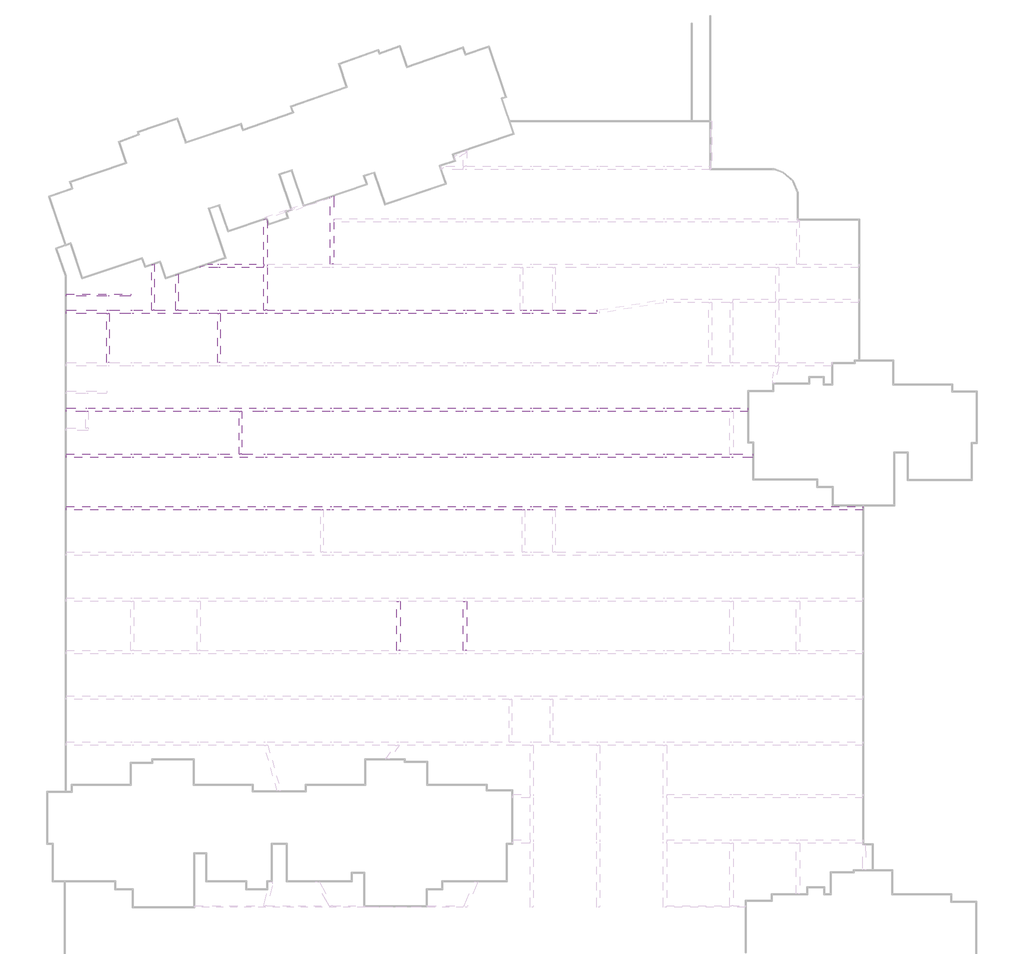
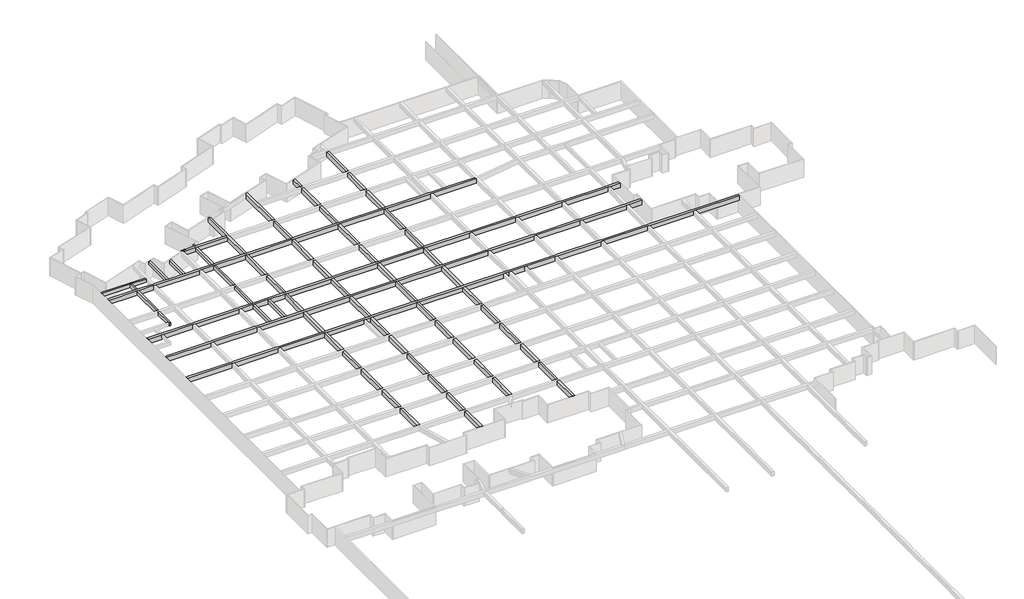
# One storey, part 13 of 14: 15 beams.
"""IFC4 building model written with IfcOpenShell, lengths in millimetres."""

from ifc_helpers import new_model, si_unit, frame, origin, place, context, project, spatial, polyline, outline, extrude, faceted_brep, element, save

model = new_model("IFC4")

# Units and contexts
model_context = context("Model", 3, world=origin())
ifc_project = project(units=[si_unit("LENGTHUNIT", "METRE", prefix="MILLI")], contexts=[model_context])

# Site, building, storey
site = spatial("IfcSite", under=ifc_project)
building = spatial("IfcBuilding", under=site)
storey = spatial("IfcBuildingStorey", under=building, Name="户型图", Elevation=0.0)

# Beams
placement = place(None, origin())
element("IfcBeam", 1, ObjectType="混凝土 - 矩形梁 : KL_beam", at=placement, inside=storey, context=model_context, shape_type="Brep", body=[
    faceted_brep([(-594019.2557706, -38859.4327531, 3300.0), (-594019.2557706, -39259.4327531, 3300.0), (-589117.6529954, -39259.4327531, 3300.0), (-588817.6529954, -39259.4327531, 3300.0), (-586267.6529954, -39259.4327531, 3300.0), (-585867.6529954, -39259.4327531, 3300.0), (-578267.6529954, -39259.4327531, 3300.0), (-577867.6529954, -39259.4327531, 3300.0), (-575817.6529954, -39259.4327531, 3300.0), (-575517.6529954, -39259.4327531, 3300.0), (-570267.6529954, -39259.4327531, 3300.0), (-569867.6529954, -39259.4327531, 3300.0), (-562267.6529954, -39259.4327531, 3300.0), (-561867.6529954, -39259.4327531, 3300.0), (-554267.6529954, -39259.4327531, 3300.0), (-553867.6529954, -39259.4327531, 3300.0), (-546267.6529954, -39259.4327531, 3300.0), (-545867.6529954, -39259.4327531, 3300.0), (-538267.6529954, -39259.4327531, 3300.0), (-537867.6529954, -39259.4327531, 3300.0), (-530267.6529954, -39259.4327531, 3300.0), (-530267.6529954, -38859.4327531, 3300.0), (-535217.6529954, -38859.4327531, 3300.0), (-535517.6529954, -38859.4327531, 3300.0), (-537867.6529954, -38859.4327531, 3300.0), (-538267.6529954, -38859.4327531, 3300.0), (-539117.6529954, -38859.4327531, 3300.0), (-539417.6529954, -38859.4327531, 3300.0), (-545867.6529954, -38859.4327531, 3300.0), (-546267.6529954, -38859.4327531, 3300.0), (-553867.6529954, -38859.4327531, 3300.0), (-554267.6529954, -38859.4327531, 3300.0), (-561867.6529954, -38859.4327531, 3300.0), (-562267.6529954, -38859.4327531, 3300.0), (-569867.6529954, -38859.4327531, 3300.0), (-570267.6529954, -38859.4327531, 3300.0), (-575517.6529954, -38859.4327531, 3300.0), (-575817.6529954, -38859.4327531, 3300.0), (-577867.6529954, -38859.4327531, 3300.0), (-578267.6529954, -38859.4327531, 3300.0), (-580530.3460998, -38859.4327531, 3300.0), (-580830.3460998, -38859.4327531, 3300.0), (-583417.6956186, -38859.4327531, 3300.0), (-583717.6956186, -38859.4327531, 3300.0), (-585867.6529954, -38859.4327531, 3300.0), (-586267.6529954, -38859.4327531, 3300.0), (-588817.6529954, -38859.4327531, 3300.0), (-589117.6529954, -38859.4327531, 3300.0), (-594019.2557706, -39259.4327531, 2500.0), (-586267.6529954, -39259.4327531, 2500.0), (-585867.6529954, -39259.4327531, 2500.0), (-578267.6529954, -39259.4327531, 2500.0), (-577867.6529954, -39259.4327531, 2500.0), (-570267.6529954, -39259.4327531, 2500.0), (-569867.6529954, -39259.4327531, 2500.0), (-562267.6529954, -39259.4327531, 2500.0), (-561867.6529954, -39259.4327531, 2500.0), (-554267.6529954, -39259.4327531, 2500.0), (-553867.6529954, -39259.4327531, 2500.0), (-546267.6529954, -39259.4327531, 2500.0), (-545867.6529954, -39259.4327531, 2500.0), (-538267.6529954, -39259.4327531, 2500.0), (-537867.6529954, -39259.4327531, 2500.0), (-530267.6529954, -39259.4327531, 2500.0), (-594019.2557706, -38859.4327531, 2500.0), (-586267.6529954, -38859.4327531, 2500.0), (-585867.6529954, -38859.4327531, 2500.0), (-578267.6529954, -38859.4327531, 2500.0), (-577867.6529954, -38859.4327531, 2500.0), (-570267.6529954, -38859.4327531, 2500.0), (-569867.6529954, -38859.4327531, 2500.0), (-562267.6529954, -38859.4327531, 2500.0), (-561867.6529954, -38859.4327531, 2500.0), (-554267.6529954, -38859.4327531, 2500.0), (-553867.6529954, -38859.4327531, 2500.0), (-546267.6529954, -38859.4327531, 2500.0), (-545867.6529954, -38859.4327531, 2500.0), (-538267.6529954, -38859.4327531, 2500.0), (-537867.6529954, -38859.4327531, 2500.0), (-530267.6529954, -38859.4327531, 2500.0)], [[[0, 1, 2, 3, 4, 5, 6, 7, 8, 9, 10, 11, 12, 13, 14, 15, 16, 17, 18, 19, 20, 21, 22, 23, 24, 25, 26, 27, 28, 29, 30, 31, 32, 33, 34, 35, 36, 37, 38, 39, 40, 41, 42, 43, 44, 45, 46, 47]], [[1, 48, 49, 50, 51, 52, 53, 54, 55, 56, 57, 58, 59, 60, 61, 62, 63, 20, 19, 18, 17, 16, 15, 14, 13, 12, 11, 10, 9, 8, 7, 6, 5, 4, 3, 2]], [[48, 64, 65, 66, 67, 68, 69, 70, 71, 72, 73, 74, 75, 76, 77, 78, 79, 63, 62, 61, 60, 59, 58, 57, 56, 55, 54, 53, 52, 51, 50, 49]], [[64, 0, 47, 46, 45, 44, 43, 42, 41, 40, 39, 38, 37, 36, 35, 34, 33, 32, 31, 30, 29, 28, 27, 26, 25, 24, 23, 22, 21, 79, 78, 77, 76, 75, 74, 73, 72, 71, 70, 69, 68, 67, 66, 65]], [[1, 0, 64, 48]], [[21, 20, 63, 79]]]),
])
element("IfcBeam", 2, ObjectType="混凝土 - 矩形梁 : KL_beam", at=placement, inside=storey, context=model_context, shape_type="Brep", body=[
    faceted_brep([(-594019.2557706, -56159.4327531, 3300.0), (-594019.2557706, -56559.4327531, 3300.0), (-586267.6529954, -56559.4327531, 3300.0), (-585867.6529954, -56559.4327531, 3300.0), (-578267.6529954, -56559.4327531, 3300.0), (-577867.6529954, -56559.4327531, 3300.0), (-570267.6529954, -56559.4327531, 3300.0), (-569867.6529954, -56559.4327531, 3300.0), (-562267.6529954, -56559.4327531, 3300.0), (-561867.6529954, -56559.4327531, 3300.0), (-554267.6529954, -56559.4327531, 3300.0), (-553867.6529954, -56559.4327531, 3300.0), (-546267.6529954, -56559.4327531, 3300.0), (-545867.6529954, -56559.4327531, 3300.0), (-538267.6529954, -56559.4327531, 3300.0), (-537867.6529954, -56559.4327531, 3300.0), (-530267.6529954, -56559.4327531, 3300.0), (-529867.6529954, -56559.4327531, 3300.0), (-522267.6529954, -56559.4327531, 3300.0), (-521867.6529954, -56559.4327531, 3300.0), (-514267.6529954, -56559.4327531, 3300.0), (-513867.6529954, -56559.4327531, 3300.0), (-511515.1621146, -56559.4327531, 3300.0), (-511515.1621146, -56159.4327531, 3300.0), (-513867.6529954, -56159.4327531, 3300.0), (-514267.6529954, -56159.4327531, 3300.0), (-521867.6529954, -56159.4327531, 3300.0), (-522267.6529954, -56159.4327531, 3300.0), (-529867.6529954, -56159.4327531, 3300.0), (-530267.6529954, -56159.4327531, 3300.0), (-537867.6529954, -56159.4327531, 3300.0), (-538267.6529954, -56159.4327531, 3300.0), (-545867.6529954, -56159.4327531, 3300.0), (-546267.6529954, -56159.4327531, 3300.0), (-553867.6529954, -56159.4327531, 3300.0), (-554267.6529954, -56159.4327531, 3300.0), (-561867.6529954, -56159.4327531, 3300.0), (-562267.6529954, -56159.4327531, 3300.0), (-569867.6529954, -56159.4327531, 3300.0), (-570267.6529954, -56159.4327531, 3300.0), (-572917.6529954, -56159.4327531, 3300.0), (-573217.6529954, -56159.4327531, 3300.0), (-575517.6529954, -56159.4327531, 3300.0), (-575817.6529954, -56159.4327531, 3300.0), (-577867.6529954, -56159.4327531, 3300.0), (-578267.6529954, -56159.4327531, 3300.0), (-585867.6529954, -56159.4327531, 3300.0), (-586267.6529954, -56159.4327531, 3300.0), (-594019.2557706, -56559.4327531, 2500.0), (-586267.6529954, -56559.4327531, 2500.0), (-585867.6529954, -56559.4327531, 2500.0), (-578267.6529954, -56559.4327531, 2500.0), (-577867.6529954, -56559.4327531, 2500.0), (-570267.6529954, -56559.4327531, 2500.0), (-569867.6529954, -56559.4327531, 2500.0), (-562267.6529954, -56559.4327531, 2500.0), (-561867.6529954, -56559.4327531, 2500.0), (-554267.6529954, -56559.4327531, 2500.0), (-553867.6529954, -56559.4327531, 2500.0), (-546267.6529954, -56559.4327531, 2500.0), (-545867.6529954, -56559.4327531, 2500.0), (-538267.6529954, -56559.4327531, 2500.0), (-537867.6529954, -56559.4327531, 2500.0), (-530267.6529954, -56559.4327531, 2500.0), (-529867.6529954, -56559.4327531, 2500.0), (-522267.6529954, -56559.4327531, 2500.0), (-521867.6529954, -56559.4327531, 2500.0), (-514267.6529954, -56559.4327531, 2500.0), (-513867.6529954, -56559.4327531, 2500.0), (-511515.1621146, -56559.4327531, 2500.0), (-594019.2557706, -56159.4327531, 2500.0), (-586267.6529954, -56159.4327531, 2500.0), (-585867.6529954, -56159.4327531, 2500.0), (-578267.6529954, -56159.4327531, 2500.0), (-577867.6529954, -56159.4327531, 2500.0), (-570267.6529954, -56159.4327531, 2500.0), (-569867.6529954, -56159.4327531, 2500.0), (-562267.6529954, -56159.4327531, 2500.0), (-561867.6529954, -56159.4327531, 2500.0), (-554267.6529954, -56159.4327531, 2500.0), (-553867.6529954, -56159.4327531, 2500.0), (-546267.6529954, -56159.4327531, 2500.0), (-545867.6529954, -56159.4327531, 2500.0), (-538267.6529954, -56159.4327531, 2500.0), (-537867.6529954, -56159.4327531, 2500.0), (-530267.6529954, -56159.4327531, 2500.0), (-529867.6529954, -56159.4327531, 2500.0), (-522267.6529954, -56159.4327531, 2500.0), (-521867.6529954, -56159.4327531, 2500.0), (-514267.6529954, -56159.4327531, 2500.0), (-513867.6529954, -56159.4327531, 2500.0), (-511515.1621146, -56159.4327531, 2500.0)], [[[0, 1, 2, 3, 4, 5, 6, 7, 8, 9, 10, 11, 12, 13, 14, 15, 16, 17, 18, 19, 20, 21, 22, 23, 24, 25, 26, 27, 28, 29, 30, 31, 32, 33, 34, 35, 36, 37, 38, 39, 40, 41, 42, 43, 44, 45, 46, 47]], [[1, 48, 49, 50, 51, 52, 53, 54, 55, 56, 57, 58, 59, 60, 61, 62, 63, 64, 65, 66, 67, 68, 69, 22, 21, 20, 19, 18, 17, 16, 15, 14, 13, 12, 11, 10, 9, 8, 7, 6, 5, 4, 3, 2]], [[48, 70, 71, 72, 73, 74, 75, 76, 77, 78, 79, 80, 81, 82, 83, 84, 85, 86, 87, 88, 89, 90, 91, 69, 68, 67, 66, 65, 64, 63, 62, 61, 60, 59, 58, 57, 56, 55, 54, 53, 52, 51, 50, 49]], [[70, 0, 47, 46, 45, 44, 43, 42, 41, 40, 39, 38, 37, 36, 35, 34, 33, 32, 31, 30, 29, 28, 27, 26, 25, 24, 23, 91, 90, 89, 88, 87, 86, 85, 84, 83, 82, 81, 80, 79, 78, 77, 76, 75, 74, 73, 72, 71]], [[1, 0, 70, 48]], [[23, 22, 69, 91]]]),
])
element("IfcBeam", 3, ObjectType="混凝土 - 矩形梁 : KL_beam", at=placement, inside=storey, context=model_context, shape_type="Brep", body=[
    faceted_brep([(-594019.2557706, -50659.4327531, 3300.0), (-594019.2557706, -51059.4327531, 3300.0), (-591673.454383, -51059.4327531, 3300.0), (-591373.454383, -51059.4327531, 3300.0), (-586267.6529954, -51059.4327531, 3300.0), (-585867.6529954, -51059.4327531, 3300.0), (-578267.6529954, -51059.4327531, 3300.0), (-577867.6529954, -51059.4327531, 3300.0), (-575817.6529954, -51059.4327531, 3300.0), (-575517.6529954, -51059.4327531, 3300.0), (-573217.6529954, -51059.4327531, 3300.0), (-572917.6529954, -51059.4327531, 3300.0), (-570267.6529954, -51059.4327531, 3300.0), (-569867.6529954, -51059.4327531, 3300.0), (-562267.6529954, -51059.4327531, 3300.0), (-561867.6529954, -51059.4327531, 3300.0), (-554267.6529954, -51059.4327531, 3300.0), (-553867.6529954, -51059.4327531, 3300.0), (-546267.6529954, -51059.4327531, 3300.0), (-545867.6529954, -51059.4327531, 3300.0), (-538267.6529954, -51059.4327531, 3300.0), (-537867.6529954, -51059.4327531, 3300.0), (-530267.6529954, -51059.4327531, 3300.0), (-529867.6529954, -51059.4327531, 3300.0), (-522267.6529954, -51059.4327531, 3300.0), (-521867.6529954, -51059.4327531, 3300.0), (-514267.6529954, -51059.4327531, 3300.0), (-513867.6529954, -51059.4327531, 3300.0), (-512115.1621146, -51059.4327531, 3300.0), (-512115.1621146, -50659.4327531, 3300.0), (-513867.6529954, -50659.4327531, 3300.0), (-514267.6529954, -50659.4327531, 3300.0), (-521867.6529954, -50659.4327531, 3300.0), (-522267.6529954, -50659.4327531, 3300.0), (-529867.6529954, -50659.4327531, 3300.0), (-530267.6529954, -50659.4327531, 3300.0), (-537867.6529954, -50659.4327531, 3300.0), (-538267.6529954, -50659.4327531, 3300.0), (-545867.6529954, -50659.4327531, 3300.0), (-546267.6529954, -50659.4327531, 3300.0), (-553867.6529954, -50659.4327531, 3300.0), (-554267.6529954, -50659.4327531, 3300.0), (-561867.6529954, -50659.4327531, 3300.0), (-562267.6529954, -50659.4327531, 3300.0), (-569867.6529954, -50659.4327531, 3300.0), (-570267.6529954, -50659.4327531, 3300.0), (-575517.6529954, -50659.4327531, 3300.0), (-575817.6529954, -50659.4327531, 3300.0), (-577867.6529954, -50659.4327531, 3300.0), (-578267.6529954, -50659.4327531, 3300.0), (-585867.6529954, -50659.4327531, 3300.0), (-586267.6529954, -50659.4327531, 3300.0), (-591373.454383, -50659.4327531, 3300.0), (-591673.454383, -50659.4327531, 3300.0), (-594019.2557706, -51059.4327531, 2500.0), (-586267.6529954, -51059.4327531, 2500.0), (-585867.6529954, -51059.4327531, 2500.0), (-578267.6529954, -51059.4327531, 2500.0), (-577867.6529954, -51059.4327531, 2500.0), (-570267.6529954, -51059.4327531, 2500.0), (-569867.6529954, -51059.4327531, 2500.0), (-562267.6529954, -51059.4327531, 2500.0), (-561867.6529954, -51059.4327531, 2500.0), (-554267.6529954, -51059.4327531, 2500.0), (-553867.6529954, -51059.4327531, 2500.0), (-546267.6529954, -51059.4327531, 2500.0), (-545867.6529954, -51059.4327531, 2500.0), (-538267.6529954, -51059.4327531, 2500.0), (-537867.6529954, -51059.4327531, 2500.0), (-530267.6529954, -51059.4327531, 2500.0), (-529867.6529954, -51059.4327531, 2500.0), (-522267.6529954, -51059.4327531, 2500.0), (-521867.6529954, -51059.4327531, 2500.0), (-514267.6529954, -51059.4327531, 2500.0), (-513867.6529954, -51059.4327531, 2500.0), (-512115.1621146, -51059.4327531, 2500.0), (-594019.2557706, -50659.4327531, 2500.0), (-586267.6529954, -50659.4327531, 2500.0), (-585867.6529954, -50659.4327531, 2500.0), (-578267.6529954, -50659.4327531, 2500.0), (-577867.6529954, -50659.4327531, 2500.0), (-570267.6529954, -50659.4327531, 2500.0), (-569867.6529954, -50659.4327531, 2500.0), (-562267.6529954, -50659.4327531, 2500.0), (-561867.6529954, -50659.4327531, 2500.0), (-554267.6529954, -50659.4327531, 2500.0), (-553867.6529954, -50659.4327531, 2500.0), (-546267.6529954, -50659.4327531, 2500.0), (-545867.6529954, -50659.4327531, 2500.0), (-538267.6529954, -50659.4327531, 2500.0), (-537867.6529954, -50659.4327531, 2500.0), (-530267.6529954, -50659.4327531, 2500.0), (-529867.6529954, -50659.4327531, 2500.0), (-522267.6529954, -50659.4327531, 2500.0), (-521867.6529954, -50659.4327531, 2500.0), (-514267.6529954, -50659.4327531, 2500.0), (-513867.6529954, -50659.4327531, 2500.0), (-512115.1621146, -50659.4327531, 2500.0)], [[[0, 1, 2, 3, 4, 5, 6, 7, 8, 9, 10, 11, 12, 13, 14, 15, 16, 17, 18, 19, 20, 21, 22, 23, 24, 25, 26, 27, 28, 29, 30, 31, 32, 33, 34, 35, 36, 37, 38, 39, 40, 41, 42, 43, 44, 45, 46, 47, 48, 49, 50, 51, 52, 53]], [[1, 54, 55, 56, 57, 58, 59, 60, 61, 62, 63, 64, 65, 66, 67, 68, 69, 70, 71, 72, 73, 74, 75, 28, 27, 26, 25, 24, 23, 22, 21, 20, 19, 18, 17, 16, 15, 14, 13, 12, 11, 10, 9, 8, 7, 6, 5, 4, 3, 2]], [[54, 76, 77, 78, 79, 80, 81, 82, 83, 84, 85, 86, 87, 88, 89, 90, 91, 92, 93, 94, 95, 96, 97, 75, 74, 73, 72, 71, 70, 69, 68, 67, 66, 65, 64, 63, 62, 61, 60, 59, 58, 57, 56, 55]], [[76, 0, 53, 52, 51, 50, 49, 48, 47, 46, 45, 44, 43, 42, 41, 40, 39, 38, 37, 36, 35, 34, 33, 32, 31, 30, 29, 97, 96, 95, 94, 93, 92, 91, 90, 89, 88, 87, 86, 85, 84, 83, 82, 81, 80, 79, 78, 77]], [[1, 0, 76, 54]], [[29, 28, 75, 97]]]),
])
element("IfcBeam", 4, ObjectType="混凝土 - 矩形梁 : KL_beam", at=placement, inside=storey, context=model_context, shape_type="Brep", body=[
    faceted_brep([(-594019.2557706, -62459.4327531, 3300.0), (-594019.2557706, -62859.4327531, 3300.0), (-586267.6529954, -62859.4327531, 3300.0), (-585867.6529954, -62859.4327531, 3300.0), (-578267.6529954, -62859.4327531, 3300.0), (-577867.6529954, -62859.4327531, 3300.0), (-570267.6529954, -62859.4327531, 3300.0), (-569867.6529954, -62859.4327531, 3300.0), (-563417.6529954, -62859.4327531, 3300.0), (-563117.6529954, -62859.4327531, 3300.0), (-562267.6529954, -62859.4327531, 3300.0), (-561867.6529954, -62859.4327531, 3300.0), (-554267.6529954, -62859.4327531, 3300.0), (-553867.6529954, -62859.4327531, 3300.0), (-546267.6529954, -62859.4327531, 3300.0), (-545867.6529954, -62859.4327531, 3300.0), (-539217.6529954, -62859.4327531, 3300.0), (-538917.6529954, -62859.4327531, 3300.0), (-538267.6529954, -62859.4327531, 3300.0), (-537867.6529954, -62859.4327531, 3300.0), (-535517.6529954, -62859.4327531, 3300.0), (-535217.6529954, -62859.4327531, 3300.0), (-530267.6529954, -62859.4327531, 3300.0), (-529867.6529954, -62859.4327531, 3300.0), (-522267.6529954, -62859.4327531, 3300.0), (-521867.6529954, -62859.4327531, 3300.0), (-514267.6529954, -62859.4327531, 3300.0), (-513867.6529954, -62859.4327531, 3300.0), (-506267.6529954, -62859.4327531, 3300.0), (-505867.6529954, -62859.4327531, 3300.0), (-498277.6529954, -62859.4327531, 3300.0), (-498277.6529954, -62459.4327531, 3300.0), (-505867.6529954, -62459.4327531, 3300.0), (-506267.6529954, -62459.4327531, 3300.0), (-513867.6529954, -62459.4327531, 3300.0), (-514267.6529954, -62459.4327531, 3300.0), (-521867.6529954, -62459.4327531, 3300.0), (-522267.6529954, -62459.4327531, 3300.0), (-529867.6529954, -62459.4327531, 3300.0), (-530267.6529954, -62459.4327531, 3300.0), (-537867.6529954, -62459.4327531, 3300.0), (-538267.6529954, -62459.4327531, 3300.0), (-545867.6529954, -62459.4327531, 3300.0), (-546267.6529954, -62459.4327531, 3300.0), (-553867.6529954, -62459.4327531, 3300.0), (-554267.6529954, -62459.4327531, 3300.0), (-561867.6529954, -62459.4327531, 3300.0), (-562267.6529954, -62459.4327531, 3300.0), (-569867.6529954, -62459.4327531, 3300.0), (-570267.6529954, -62459.4327531, 3300.0), (-577867.6529954, -62459.4327531, 3300.0), (-578267.6529954, -62459.4327531, 3300.0), (-585867.6529954, -62459.4327531, 3300.0), (-586267.6529954, -62459.4327531, 3300.0), (-594019.2557706, -62859.4327531, 2500.0), (-586267.6529954, -62859.4327531, 2500.0), (-585867.6529954, -62859.4327531, 2500.0), (-578267.6529954, -62859.4327531, 2500.0), (-577867.6529954, -62859.4327531, 2500.0), (-570267.6529954, -62859.4327531, 2500.0), (-569867.6529954, -62859.4327531, 2500.0), (-562267.6529954, -62859.4327531, 2500.0), (-561867.6529954, -62859.4327531, 2500.0), (-554267.6529954, -62859.4327531, 2500.0), (-553867.6529954, -62859.4327531, 2500.0), (-546267.6529954, -62859.4327531, 2500.0), (-545867.6529954, -62859.4327531, 2500.0), (-538267.6529954, -62859.4327531, 2500.0), (-537867.6529954, -62859.4327531, 2500.0), (-530267.6529954, -62859.4327531, 2500.0), (-529867.6529954, -62859.4327531, 2500.0), (-522267.6529954, -62859.4327531, 2500.0), (-521867.6529954, -62859.4327531, 2500.0), (-514267.6529954, -62859.4327531, 2500.0), (-513867.6529954, -62859.4327531, 2500.0), (-506267.6529954, -62859.4327531, 2500.0), (-505867.6529954, -62859.4327531, 2500.0), (-498277.6529954, -62859.4327531, 2500.0), (-594019.2557706, -62459.4327531, 2500.0), (-586267.6529954, -62459.4327531, 2500.0), (-585867.6529954, -62459.4327531, 2500.0), (-578267.6529954, -62459.4327531, 2500.0), (-577867.6529954, -62459.4327531, 2500.0), (-570267.6529954, -62459.4327531, 2500.0), (-569867.6529954, -62459.4327531, 2500.0), (-562267.6529954, -62459.4327531, 2500.0), (-561867.6529954, -62459.4327531, 2500.0), (-554267.6529954, -62459.4327531, 2500.0), (-553867.6529954, -62459.4327531, 2500.0), (-546267.6529954, -62459.4327531, 2500.0), (-545867.6529954, -62459.4327531, 2500.0), (-538267.6529954, -62459.4327531, 2500.0), (-537867.6529954, -62459.4327531, 2500.0), (-530267.6529954, -62459.4327531, 2500.0), (-529867.6529954, -62459.4327531, 2500.0), (-522267.6529954, -62459.4327531, 2500.0), (-521867.6529954, -62459.4327531, 2500.0), (-514267.6529954, -62459.4327531, 2500.0), (-513867.6529954, -62459.4327531, 2500.0), (-506267.6529954, -62459.4327531, 2500.0), (-505867.6529954, -62459.4327531, 2500.0), (-498277.6529954, -62459.4327531, 2500.0)], [[[0, 1, 2, 3, 4, 5, 6, 7, 8, 9, 10, 11, 12, 13, 14, 15, 16, 17, 18, 19, 20, 21, 22, 23, 24, 25, 26, 27, 28, 29, 30, 31, 32, 33, 34, 35, 36, 37, 38, 39, 40, 41, 42, 43, 44, 45, 46, 47, 48, 49, 50, 51, 52, 53]], [[1, 54, 55, 56, 57, 58, 59, 60, 61, 62, 63, 64, 65, 66, 67, 68, 69, 70, 71, 72, 73, 74, 75, 76, 77, 30, 29, 28, 27, 26, 25, 24, 23, 22, 21, 20, 19, 18, 17, 16, 15, 14, 13, 12, 11, 10, 9, 8, 7, 6, 5, 4, 3, 2]], [[54, 78, 79, 80, 81, 82, 83, 84, 85, 86, 87, 88, 89, 90, 91, 92, 93, 94, 95, 96, 97, 98, 99, 100, 101, 77, 76, 75, 74, 73, 72, 71, 70, 69, 68, 67, 66, 65, 64, 63, 62, 61, 60, 59, 58, 57, 56, 55]], [[78, 0, 53, 52, 51, 50, 49, 48, 47, 46, 45, 44, 43, 42, 41, 40, 39, 38, 37, 36, 35, 34, 33, 32, 31, 101, 100, 99, 98, 97, 96, 95, 94, 93, 92, 91, 90, 89, 88, 87, 86, 85, 84, 83, 82, 81, 80, 79]], [[1, 0, 78, 54]], [[31, 30, 77, 101]]]),
])
element("IfcBeam", 5, ObjectType="混凝土 - 矩形梁 : KL_beam", at=placement, inside=storey, context=model_context, shape_type="Brep", body=[
    faceted_brep([(-569950.4085273, -27888.1137818, 3300.0), (-570267.6529954, -27994.502473, 3300.0), (-570267.6529954, -33359.4327531, 3300.0), (-570267.6529954, -33759.4327531, 3300.0), (-570267.6529954, -38859.4327531, 3300.0), (-569867.6529954, -38859.4327531, 3300.0), (-569867.6529954, -33759.4327531, 3300.0), (-569867.6529954, -33359.4327531, 3300.0), (-569867.6529954, -28133.2700068, 3300.0), (-569867.6529954, -28133.2700068, 2500.0), (-569867.6529954, -38859.4327531, 2500.0), (-569867.6529954, -33759.4327531, 2500.0), (-569867.6529954, -33359.4327531, 2500.0), (-570267.6529954, -27994.502473, 2500.0), (-569950.4085273, -27888.1137818, 2500.0), (-570267.6529954, -38859.4327531, 2500.0), (-570267.6529954, -33759.4327531, 2500.0), (-570267.6529954, -33359.4327531, 2500.0)], [[[0, 1, 2, 3, 4, 5, 6, 7, 8]], [[9, 8, 7, 6, 5, 10, 11, 12]], [[13, 14, 9, 12, 11, 10, 15, 16, 17]], [[1, 13, 17, 16, 15, 4, 3, 2]], [[13, 1, 0, 14]], [[14, 0, 8, 9]], [[4, 15, 10, 5]]]),
    faceted_brep([(-570267.6529954, -90759.4327531, 3300.0), (-570267.6529954, -90759.4327531, 2500.0), (-569867.6529954, -90759.4327531, 2500.0), (-569867.6529954, -90759.4327531, 3300.0), (-570267.6529954, -85659.4327531, 2500.0), (-570267.6529954, -85659.4327531, 3300.0), (-569867.6529954, -85659.4327531, 3300.0), (-569867.6529954, -85659.4327531, 2500.0)], [[[0, 1, 2, 3]], [[4, 5, 6, 7]], [[1, 0, 5, 4]], [[0, 3, 6, 5]], [[3, 2, 7, 6]], [[2, 1, 4, 7]]]),
    faceted_brep([(-570267.6529954, -39259.4327531, 2500.0), (-570267.6529954, -39259.4327531, 3300.0), (-569867.6529954, -39259.4327531, 3300.0), (-569867.6529954, -39259.4327531, 2500.0), (-570267.6529954, -45159.4327531, 2500.0), (-570267.6529954, -45159.4327531, 3300.0), (-569867.6529954, -45159.4327531, 2500.0), (-569867.6529954, -45159.4327531, 3300.0)], [[[0, 1, 2, 3]], [[1, 0, 4, 5]], [[5, 4, 6, 7]], [[2, 1, 5, 7]], [[3, 2, 7, 6]], [[0, 3, 6, 4]]]),
    faceted_brep([(-570267.6529954, -45559.4327531, 2500.0), (-570267.6529954, -45559.4327531, 3300.0), (-569867.6529954, -45559.4327531, 3300.0), (-569867.6529954, -45559.4327531, 2500.0), (-570267.6529954, -50659.4327531, 2500.0), (-570267.6529954, -50659.4327531, 3300.0), (-569867.6529954, -50659.4327531, 2500.0), (-569867.6529954, -50659.4327531, 3300.0)], [[[0, 1, 2, 3]], [[1, 0, 4, 5]], [[5, 4, 6, 7]], [[2, 1, 5, 7]], [[3, 2, 7, 6]], [[0, 3, 6, 4]]]),
    faceted_brep([(-570267.6529954, -56559.4327531, 2500.0), (-570267.6529954, -56559.4327531, 3300.0), (-569867.6529954, -56559.4327531, 3300.0), (-569867.6529954, -56559.4327531, 2500.0), (-570267.6529954, -62459.4327531, 2500.0), (-570267.6529954, -62459.4327531, 3300.0), (-569867.6529954, -62459.4327531, 2500.0), (-569867.6529954, -62459.4327531, 3300.0)], [[[0, 1, 2, 3]], [[1, 0, 4, 5]], [[5, 4, 6, 7]], [[2, 1, 5, 7]], [[3, 2, 7, 6]], [[0, 3, 6, 4]]]),
    faceted_brep([(-570267.6529954, -56159.4327531, 3300.0), (-570267.6529954, -56159.4327531, 2500.0), (-569867.6529954, -56159.4327531, 2500.0), (-569867.6529954, -56159.4327531, 3300.0), (-570267.6529954, -51059.4327531, 2500.0), (-570267.6529954, -51059.4327531, 3300.0), (-569867.6529954, -51059.4327531, 3300.0), (-569867.6529954, -51059.4327531, 2500.0)], [[[0, 1, 2, 3]], [[4, 5, 6, 7]], [[1, 0, 5, 4]], [[0, 3, 6, 5]], [[3, 2, 7, 6]], [[2, 1, 4, 7]]]),
    faceted_brep([(-570267.6529954, -62859.4327531, 2500.0), (-570267.6529954, -62859.4327531, 3300.0), (-569867.6529954, -62859.4327531, 3300.0), (-569867.6529954, -62859.4327531, 2500.0), (-570267.6529954, -67959.4327531, 2500.0), (-570267.6529954, -67959.4327531, 3300.0), (-569867.6529954, -67959.4327531, 2500.0), (-569867.6529954, -67959.4327531, 3300.0)], [[[0, 1, 2, 3]], [[1, 0, 4, 5]], [[5, 4, 6, 7]], [[2, 1, 5, 7]], [[3, 2, 7, 6]], [[0, 3, 6, 4]]]),
    faceted_brep([(-570267.6529954, -68359.4327531, 2500.0), (-570267.6529954, -68359.4327531, 3300.0), (-569867.6529954, -68359.4327531, 3300.0), (-569867.6529954, -68359.4327531, 2500.0), (-570267.6529954, -73459.4327531, 2500.0), (-570267.6529954, -73459.4327531, 3300.0), (-569867.6529954, -73459.4327531, 2500.0), (-569867.6529954, -73459.4327531, 3300.0)], [[[0, 1, 2, 3]], [[1, 0, 4, 5]], [[5, 4, 6, 7]], [[2, 1, 5, 7]], [[3, 2, 7, 6]], [[0, 3, 6, 4]]]),
    faceted_brep([(-570267.6529954, -73859.4327531, 2500.0), (-570267.6529954, -73859.4327531, 3300.0), (-569867.6529954, -73859.4327531, 3300.0), (-569867.6529954, -73859.4327531, 2500.0), (-570267.6529954, -79759.4327531, 2500.0), (-570267.6529954, -79759.4327531, 3300.0), (-569867.6529954, -79759.4327531, 2500.0), (-569867.6529954, -79759.4327531, 3300.0)], [[[0, 1, 2, 3]], [[1, 0, 4, 5]], [[5, 4, 6, 7]], [[2, 1, 5, 7]], [[3, 2, 7, 6]], [[0, 3, 6, 4]]]),
    faceted_brep([(-570267.6529954, -80159.4327531, 2500.0), (-570267.6529954, -80159.4327531, 3300.0), (-569867.6529954, -80159.4327531, 3300.0), (-569867.6529954, -80159.4327531, 2500.0), (-570267.6529954, -85259.4327531, 2500.0), (-570267.6529954, -85259.4327531, 3300.0), (-569867.6529954, -85259.4327531, 2500.0), (-569867.6529954, -85259.4327531, 3300.0)], [[[0, 1, 2, 3]], [[1, 0, 4, 5]], [[5, 4, 6, 7]], [[2, 1, 5, 7]], [[3, 2, 7, 6]], [[0, 3, 6, 4]]]),
])
element("IfcBeam", 6, ObjectType="混凝土 - 矩形梁 : KL_beam", at=placement, inside=storey, context=model_context, shape_type="Brep", body=[
    faceted_brep([(-561867.6529954, -25159.8064152, 3300.0), (-562267.6529954, -25294.8313886, 3300.0), (-562267.6529954, -25442.5926439, 3300.0), (-562267.6529954, -33359.4327531, 3300.0), (-561867.6529954, -33359.4327531, 3300.0), (-561867.6529954, -28259.4327531, 3300.0), (-561867.6529954, -27859.4327531, 3300.0), (-562267.6529954, -25294.8313886, 2500.0), (-562267.6529954, -25442.5926439, 2500.0), (-562267.6529954, -33359.4327531, 2500.0), (-561867.6529954, -25159.8064152, 2500.0), (-561867.6529954, -27859.4327531, 2500.0), (-561867.6529954, -28259.4327531, 2500.0), (-561867.6529954, -33359.4327531, 2500.0)], [[[0, 1, 2, 3, 4, 5, 6]], [[1, 7, 8, 9, 3, 2]], [[7, 10, 11, 12, 13, 9, 8]], [[10, 0, 6, 5, 4, 13, 12, 11]], [[1, 0, 10, 7]], [[4, 3, 9, 13]]]),
    faceted_brep([(-561867.6529954, -95855.8355501, 3300.0), (-562267.6529954, -95855.8355501, 3300.0), (-562267.6529954, -95855.8355501, 2500.0), (-561867.6529954, -95855.8355501, 2500.0), (-561867.6529954, -91159.4327531, 3300.0), (-562267.6529954, -91159.4327531, 3300.0), (-562267.6529954, -91159.4327531, 2500.0), (-561867.6529954, -91159.4327531, 2500.0)], [[[0, 1, 2, 3]], [[1, 0, 4, 5]], [[2, 1, 5, 6]], [[3, 2, 6, 7]], [[0, 3, 7, 4]], [[5, 4, 7, 6]]]),
    faceted_brep([(-562267.6529954, -33759.4327531, 3300.0), (-561867.6529954, -33759.4327531, 3300.0), (-561867.6529954, -33759.4327531, 2500.0), (-562267.6529954, -33759.4327531, 2500.0), (-561867.6529954, -38859.4327531, 3300.0), (-562267.6529954, -38859.4327531, 3300.0), (-562267.6529954, -38859.4327531, 2500.0), (-561867.6529954, -38859.4327531, 2500.0)], [[[0, 1, 2, 3]], [[4, 5, 6, 7]], [[1, 0, 5, 4]], [[0, 3, 6, 5]], [[3, 2, 7, 6]], [[2, 1, 4, 7]]]),
    faceted_brep([(-561867.6529954, -39259.4327531, 3300.0), (-562267.6529954, -39259.4327531, 3300.0), (-562267.6529954, -45159.4327531, 3300.0), (-561867.6529954, -45159.4327531, 3300.0), (-562267.6529954, -39259.4327531, 2500.0), (-562267.6529954, -45159.4327531, 2500.0), (-561867.6529954, -39259.4327531, 2500.0), (-561867.6529954, -45159.4327531, 2500.0)], [[[0, 1, 2, 3]], [[1, 4, 5, 2]], [[4, 6, 7, 5]], [[6, 0, 3, 7]], [[1, 0, 6, 4]], [[3, 2, 5, 7]]]),
    faceted_brep([(-562267.6529954, -45559.4327531, 3300.0), (-561867.6529954, -45559.4327531, 3300.0), (-561867.6529954, -45559.4327531, 2500.0), (-562267.6529954, -45559.4327531, 2500.0), (-561867.6529954, -50659.4327531, 3300.0), (-562267.6529954, -50659.4327531, 3300.0), (-562267.6529954, -50659.4327531, 2500.0), (-561867.6529954, -50659.4327531, 2500.0)], [[[0, 1, 2, 3]], [[4, 5, 6, 7]], [[1, 0, 5, 4]], [[0, 3, 6, 5]], [[3, 2, 7, 6]], [[2, 1, 4, 7]]]),
    faceted_brep([(-561867.6529954, -56559.4327531, 3300.0), (-562267.6529954, -56559.4327531, 3300.0), (-562267.6529954, -62459.4327531, 3300.0), (-561867.6529954, -62459.4327531, 3300.0), (-562267.6529954, -56559.4327531, 2500.0), (-562267.6529954, -62459.4327531, 2500.0), (-561867.6529954, -56559.4327531, 2500.0), (-561867.6529954, -62459.4327531, 2500.0)], [[[0, 1, 2, 3]], [[1, 4, 5, 2]], [[4, 6, 7, 5]], [[6, 0, 3, 7]], [[1, 0, 6, 4]], [[3, 2, 5, 7]]]),
    faceted_brep([(-561867.6529954, -56159.4327531, 3300.0), (-562267.6529954, -56159.4327531, 3300.0), (-562267.6529954, -56159.4327531, 2500.0), (-561867.6529954, -56159.4327531, 2500.0), (-561867.6529954, -51059.4327531, 3300.0), (-562267.6529954, -51059.4327531, 3300.0), (-562267.6529954, -51059.4327531, 2500.0), (-561867.6529954, -51059.4327531, 2500.0)], [[[0, 1, 2, 3]], [[1, 0, 4, 5]], [[2, 1, 5, 6]], [[3, 2, 6, 7]], [[0, 3, 7, 4]], [[5, 4, 7, 6]]]),
    faceted_brep([(-562267.6529954, -62859.4327531, 3300.0), (-561867.6529954, -62859.4327531, 3300.0), (-561867.6529954, -62859.4327531, 2500.0), (-562267.6529954, -62859.4327531, 2500.0), (-561867.6529954, -67959.4327531, 3300.0), (-562267.6529954, -67959.4327531, 3300.0), (-562267.6529954, -67959.4327531, 2500.0), (-561867.6529954, -67959.4327531, 2500.0)], [[[0, 1, 2, 3]], [[4, 5, 6, 7]], [[1, 0, 5, 4]], [[0, 3, 6, 5]], [[3, 2, 7, 6]], [[2, 1, 4, 7]]]),
    faceted_brep([(-561867.6529954, -68359.4327531, 3300.0), (-562267.6529954, -68359.4327531, 3300.0), (-562267.6529954, -73459.4327531, 3300.0), (-561867.6529954, -73459.4327531, 3300.0), (-562267.6529954, -68359.4327531, 2500.0), (-562267.6529954, -73459.4327531, 2500.0), (-561867.6529954, -68359.4327531, 2500.0), (-561867.6529954, -73459.4327531, 2500.0)], [[[0, 1, 2, 3]], [[1, 4, 5, 2]], [[4, 6, 7, 5]], [[6, 0, 3, 7]], [[1, 0, 6, 4]], [[3, 2, 5, 7]]]),
    faceted_brep([(-562267.6529954, -73859.4327531, 3300.0), (-561867.6529954, -73859.4327531, 3300.0), (-561867.6529954, -73859.4327531, 2500.0), (-562267.6529954, -73859.4327531, 2500.0), (-561867.6529954, -79759.4327531, 3300.0), (-562267.6529954, -79759.4327531, 3300.0), (-562267.6529954, -79759.4327531, 2500.0), (-561867.6529954, -79759.4327531, 2500.0)], [[[0, 1, 2, 3]], [[4, 5, 6, 7]], [[1, 0, 5, 4]], [[0, 3, 6, 5]], [[3, 2, 7, 6]], [[2, 1, 4, 7]]]),
    faceted_brep([(-561867.6529954, -80159.4327531, 3300.0), (-562267.6529954, -80159.4327531, 3300.0), (-562267.6529954, -85259.4327531, 3300.0), (-561867.6529954, -85259.4327531, 3300.0), (-562267.6529954, -80159.4327531, 2500.0), (-562267.6529954, -85259.4327531, 2500.0), (-561867.6529954, -80159.4327531, 2500.0), (-561867.6529954, -85259.4327531, 2500.0)], [[[0, 1, 2, 3]], [[1, 4, 5, 2]], [[4, 6, 7, 5]], [[6, 0, 3, 7]], [[1, 0, 6, 4]], [[3, 2, 5, 7]]]),
    faceted_brep([(-562267.6529954, -85659.4327531, 3300.0), (-561867.6529954, -85659.4327531, 3300.0), (-561867.6529954, -85659.4327531, 2500.0), (-562267.6529954, -85659.4327531, 2500.0), (-561867.6529954, -90759.4327531, 3300.0), (-562267.6529954, -90759.4327531, 3300.0), (-562267.6529954, -90759.4327531, 2500.0), (-561867.6529954, -90759.4327531, 2500.0)], [[[0, 1, 2, 3]], [[4, 5, 6, 7]], [[1, 0, 5, 4]], [[0, 3, 6, 5]], [[3, 2, 7, 6]], [[2, 1, 4, 7]]]),
])
element("IfcBeam", 7, ObjectType="混凝土 - 矩形梁 : KL_beam", at=placement, inside=storey, context=model_context, shape_type="SweptSolid", body=[
    extrude(outline(polyline([(-554267.6529954, -85659.4327531), (-553867.6529954, -85659.4327531), (-553867.6529954, -90759.4327531), (-554267.6529954, -90759.4327531), (-554267.6529954, -85659.4327531)])), frame((0.0, 0.0, 2500.0), z_axis=(0.0, 0.0, 1.0), x_axis=(1.0, 0.0, 0.0)), (0.0, 0.0, 1.0), 800.0),
    extrude(outline(polyline([(-554267.6529954, -25750.3756122), (-553867.6529954, -25615.3506388), (-553867.6529954, -27859.4327531), (-554267.6529954, -27859.4327531), (-554267.6529954, -25750.3756122)])), frame((0.0, 0.0, 2500.0), z_axis=(0.0, 0.0, 1.0), x_axis=(1.0, 0.0, 0.0)), (0.0, 0.0, 1.0), 800.0),
    extrude(outline(polyline([(-554267.6529954, -33759.4327531), (-553867.6529954, -33759.4327531), (-553867.6529954, -38859.4327531), (-554267.6529954, -38859.4327531), (-554267.6529954, -33759.4327531)])), frame((0.0, 0.0, 2500.0), z_axis=(0.0, 0.0, 1.0), x_axis=(1.0, 0.0, 0.0)), (0.0, 0.0, 1.0), 800.0),
    extrude(outline(polyline([(-553867.6529954, -33359.4327531), (-554267.6529954, -33359.4327531), (-554267.6529954, -28259.4327531), (-553867.6529954, -28259.4327531), (-553867.6529954, -33359.4327531)])), frame((0.0, 0.0, 2500.0), z_axis=(0.0, 0.0, 1.0), x_axis=(1.0, 0.0, 0.0)), (0.0, 0.0, 1.0), 800.0),
    extrude(outline(polyline([(-554267.6529954, -39259.4327531), (-553867.6529954, -39259.4327531), (-553867.6529954, -45159.4327531), (-554267.6529954, -45159.4327531), (-554267.6529954, -39259.4327531)])), frame((0.0, 0.0, 2500.0), z_axis=(0.0, 0.0, 1.0), x_axis=(1.0, 0.0, 0.0)), (0.0, 0.0, 1.0), 800.0),
    extrude(outline(polyline([(-554267.6529954, -45559.4327531), (-553867.6529954, -45559.4327531), (-553867.6529954, -50659.4327531), (-554267.6529954, -50659.4327531), (-554267.6529954, -45559.4327531)])), frame((0.0, 0.0, 2500.0), z_axis=(0.0, 0.0, 1.0), x_axis=(1.0, 0.0, 0.0)), (0.0, 0.0, 1.0), 800.0),
    extrude(outline(polyline([(-554267.6529954, -56559.4327531), (-553867.6529954, -56559.4327531), (-553867.6529954, -62459.4327531), (-554267.6529954, -62459.4327531), (-554267.6529954, -56559.4327531)])), frame((0.0, 0.0, 2500.0), z_axis=(0.0, 0.0, 1.0), x_axis=(1.0, 0.0, 0.0)), (0.0, 0.0, 1.0), 800.0),
    extrude(outline(polyline([(-553867.6529954, -56159.4327531), (-554267.6529954, -56159.4327531), (-554267.6529954, -51059.4327531), (-553867.6529954, -51059.4327531), (-553867.6529954, -56159.4327531)])), frame((0.0, 0.0, 2500.0), z_axis=(0.0, 0.0, 1.0), x_axis=(1.0, 0.0, 0.0)), (0.0, 0.0, 1.0), 800.0),
    extrude(outline(polyline([(-554267.6529954, -62859.4327531), (-553867.6529954, -62859.4327531), (-553867.6529954, -67959.4327531), (-554267.6529954, -67959.4327531), (-554267.6529954, -62859.4327531)])), frame((0.0, 0.0, 2500.0), z_axis=(0.0, 0.0, 1.0), x_axis=(1.0, 0.0, 0.0)), (0.0, 0.0, 1.0), 800.0),
    extrude(outline(polyline([(-554267.6529954, -68359.4327531), (-553867.6529954, -68359.4327531), (-553867.6529954, -73459.4327531), (-554267.6529954, -73459.4327531), (-554267.6529954, -68359.4327531)])), frame((0.0, 0.0, 2500.0), z_axis=(0.0, 0.0, 1.0), x_axis=(1.0, 0.0, 0.0)), (0.0, 0.0, 1.0), 800.0),
    extrude(outline(polyline([(-554267.6529954, -73859.4327531), (-553867.6529954, -73859.4327531), (-553867.6529954, -79759.4327531), (-554267.6529954, -79759.4327531), (-554267.6529954, -73859.4327531)])), frame((0.0, 0.0, 2500.0), z_axis=(0.0, 0.0, 1.0), x_axis=(1.0, 0.0, 0.0)), (0.0, 0.0, 1.0), 800.0),
    extrude(outline(polyline([(-554267.6529954, -80159.4327531), (-553867.6529954, -80159.4327531), (-553867.6529954, -85259.4327531), (-554267.6529954, -85259.4327531), (-554267.6529954, -80159.4327531)])), frame((0.0, 0.0, 2500.0), z_axis=(0.0, 0.0, 1.0), x_axis=(1.0, 0.0, 0.0)), (0.0, 0.0, 1.0), 800.0),
])
element("IfcBeam", 8, ObjectType="混凝土 - 矩形梁 : KL_beam", at=placement, inside=storey, context=model_context, shape_type="SweptSolid", body=[
    extrude(outline(polyline([(-546267.6529954, -21959.4327531), (-545867.6529954, -21959.4327531), (-545867.6529954, -27859.4327531), (-546267.6529954, -27859.4327531), (-546267.6529954, -21959.4327531)])), frame((0.0, 0.0, 2500.0), z_axis=(0.0, 0.0, 1.0), x_axis=(1.0, 0.0, 0.0)), (0.0, 0.0, 1.0), 800.0),
    extrude(outline(polyline([(-545867.6529954, -95855.8355501), (-546267.6529954, -95855.8355501), (-546267.6529954, -91159.4327531), (-545867.6529954, -91159.4327531), (-545867.6529954, -95855.8355501)])), frame((0.0, 0.0, 2500.0), z_axis=(0.0, 0.0, 1.0), x_axis=(1.0, 0.0, 0.0)), (0.0, 0.0, 1.0), 800.0),
    extrude(outline(polyline([(-546267.6529954, -33759.4327531), (-545867.6529954, -33759.4327531), (-545867.6529954, -38859.4327531), (-546267.6529954, -38859.4327531), (-546267.6529954, -33759.4327531)])), frame((0.0, 0.0, 2500.0), z_axis=(0.0, 0.0, 1.0), x_axis=(1.0, 0.0, 0.0)), (0.0, 0.0, 1.0), 800.0),
    extrude(outline(polyline([(-545867.6529954, -33359.4327531), (-546267.6529954, -33359.4327531), (-546267.6529954, -28259.4327531), (-545867.6529954, -28259.4327531), (-545867.6529954, -33359.4327531)])), frame((0.0, 0.0, 2500.0), z_axis=(0.0, 0.0, 1.0), x_axis=(1.0, 0.0, 0.0)), (0.0, 0.0, 1.0), 800.0),
    extrude(outline(polyline([(-546267.6529954, -39259.4327531), (-545867.6529954, -39259.4327531), (-545867.6529954, -45159.4327531), (-546267.6529954, -45159.4327531), (-546267.6529954, -39259.4327531)])), frame((0.0, 0.0, 2500.0), z_axis=(0.0, 0.0, 1.0), x_axis=(1.0, 0.0, 0.0)), (0.0, 0.0, 1.0), 800.0),
    extrude(outline(polyline([(-546267.6529954, -45559.4327531), (-545867.6529954, -45559.4327531), (-545867.6529954, -50659.4327531), (-546267.6529954, -50659.4327531), (-546267.6529954, -45559.4327531)])), frame((0.0, 0.0, 2500.0), z_axis=(0.0, 0.0, 1.0), x_axis=(1.0, 0.0, 0.0)), (0.0, 0.0, 1.0), 800.0),
    extrude(outline(polyline([(-546267.6529954, -56559.4327531), (-545867.6529954, -56559.4327531), (-545867.6529954, -62459.4327531), (-546267.6529954, -62459.4327531), (-546267.6529954, -56559.4327531)])), frame((0.0, 0.0, 2500.0), z_axis=(0.0, 0.0, 1.0), x_axis=(1.0, 0.0, 0.0)), (0.0, 0.0, 1.0), 800.0),
    extrude(outline(polyline([(-545867.6529954, -56159.4327531), (-546267.6529954, -56159.4327531), (-546267.6529954, -51059.4327531), (-545867.6529954, -51059.4327531), (-545867.6529954, -56159.4327531)])), frame((0.0, 0.0, 2500.0), z_axis=(0.0, 0.0, 1.0), x_axis=(1.0, 0.0, 0.0)), (0.0, 0.0, 1.0), 800.0),
    extrude(outline(polyline([(-546267.6529954, -62859.4327531), (-545867.6529954, -62859.4327531), (-545867.6529954, -67959.4327531), (-546267.6529954, -67959.4327531), (-546267.6529954, -62859.4327531)])), frame((0.0, 0.0, 2500.0), z_axis=(0.0, 0.0, 1.0), x_axis=(1.0, 0.0, 0.0)), (0.0, 0.0, 1.0), 800.0),
    extrude(outline(polyline([(-546267.6529954, -68359.4327531), (-545867.6529954, -68359.4327531), (-545867.6529954, -73459.4327531), (-546267.6529954, -73459.4327531), (-546267.6529954, -68359.4327531)])), frame((0.0, 0.0, 2500.0), z_axis=(0.0, 0.0, 1.0), x_axis=(1.0, 0.0, 0.0)), (0.0, 0.0, 1.0), 800.0),
    extrude(outline(polyline([(-546267.6529954, -73859.4327531), (-545867.6529954, -73859.4327531), (-545867.6529954, -79759.4327531), (-546267.6529954, -79759.4327531), (-546267.6529954, -73859.4327531)])), frame((0.0, 0.0, 2500.0), z_axis=(0.0, 0.0, 1.0), x_axis=(1.0, 0.0, 0.0)), (0.0, 0.0, 1.0), 800.0),
    extrude(outline(polyline([(-546267.6529954, -80159.4327531), (-545867.6529954, -80159.4327531), (-545867.6529954, -85259.4327531), (-546267.6529954, -85259.4327531), (-546267.6529954, -80159.4327531)])), frame((0.0, 0.0, 2500.0), z_axis=(0.0, 0.0, 1.0), x_axis=(1.0, 0.0, 0.0)), (0.0, 0.0, 1.0), 800.0),
    extrude(outline(polyline([(-546267.6529954, -85659.4327531), (-545867.6529954, -85659.4327531), (-545867.6529954, -90759.4327531), (-546267.6529954, -90759.4327531), (-546267.6529954, -85659.4327531)])), frame((0.0, 0.0, 2500.0), z_axis=(0.0, 0.0, 1.0), x_axis=(1.0, 0.0, 0.0)), (0.0, 0.0, 1.0), 800.0),
])
element("IfcBeam", 9, ObjectType="混凝土 - 矩形梁 : KL_beam", at=placement, inside=storey, context=model_context, shape_type="Brep", body=[
    faceted_brep([(-570267.6529954, -33759.4327531, 3300.0), (-570267.6529954, -33359.4327531, 3300.0), (-575517.6529954, -33359.4327531, 3300.0), (-575817.6529954, -33359.4327531, 3300.0), (-576965.1698009, -33359.4327531, 3300.0), (-577867.6529954, -33664.0771766, 3300.0), (-577867.6529954, -33759.4327531, 3300.0), (-575817.6529954, -33759.4327531, 3300.0), (-575517.6529954, -33759.4327531, 3300.0), (-570267.6529954, -33759.4327531, 2500.0), (-577867.6529954, -33759.4327531, 2500.0), (-570267.6529954, -33359.4327531, 2500.0), (-576965.1698009, -33359.4327531, 2500.0), (-577867.6529954, -33664.0771766, 2500.0)], [[[0, 1, 2, 3, 4, 5, 6, 7, 8]], [[9, 0, 8, 7, 6, 10]], [[1, 0, 9, 11]], [[4, 12, 13, 5]], [[1, 11, 12, 4, 3, 2]], [[11, 9, 10, 13, 12]], [[6, 5, 13, 10]]]),
    faceted_brep([(-578067.6529954, -33359.4327531, 2500.0), (-578067.6529954, -33359.4327531, 3300.0), (-577340.3670739, -33359.4327531, 3300.0), (-577340.3670739, -33359.4327531, 2500.0), (-578067.6529954, -33604.9371587, 2500.0), (-577867.6529954, -33537.424672, 2500.0), (-578067.6529954, -33604.9371587, 3300.0), (-577867.6529954, -33537.424672, 3300.0)], [[[0, 1, 2, 3]], [[4, 0, 3, 5]], [[6, 4, 5, 3, 2, 7]], [[1, 0, 4, 6]], [[1, 6, 7, 2]]]),
])
element("IfcBeam", 10, ObjectType="混凝土 - 矩形梁 : L_beam", at=placement, inside=storey, context=model_context, shape_type="SweptSolid", body=[
    extrude(outline(polyline([(-583717.6956186, -33422.4129717), (-583417.6956186, -33321.1442415), (-583417.6956186, -38859.4327531), (-583717.6956186, -38859.4327531), (-583717.6956186, -33422.4129717)])), frame((0.0, 0.0, 2700.0), z_axis=(0.0, 0.0, 1.0), x_axis=(1.0, 0.0, 0.0)), (0.0, 0.0, 1.0), 600.0),
])
element("IfcBeam", 11, ObjectType="混凝土 - 矩形梁 : L_beam", at=placement, inside=storey, context=model_context, shape_type="SweptSolid", body=[
    extrude(outline(polyline([(-580830.3460998, -34664.1710708), (-580530.3460998, -34562.9023408), (-580530.3460998, -38859.4327531), (-580830.3460998, -38859.4327531), (-580830.3460998, -34664.1710708)])), frame((0.0, 0.0, 2700.0), z_axis=(0.0, 0.0, 1.0), x_axis=(1.0, 0.0, 0.0)), (0.0, 0.0, 1.0), 600.0),
])
element("IfcBeam", 12, ObjectType="混凝土 - 矩形梁 : L_beam", at=placement, inside=storey, context=model_context, shape_type="Brep", body=[
    faceted_brep([(-594019.2557706, -36909.4327532, 3300.0), (-594019.2557706, -37209.4327532, 3300.0), (-589117.6529954, -37209.4327532, 3300.0), (-588817.6529954, -37209.4327532, 3300.0), (-586267.6529954, -37209.4327532, 3300.0), (-586267.6529954, -36909.4327532, 3300.0), (-594019.2557706, -37209.4327532, 2700.0), (-589117.6529954, -37209.4327532, 2700.0), (-588817.6529954, -37209.4327532, 2700.0), (-586267.6529954, -37209.4327532, 2700.0), (-594019.2557706, -36909.4327532, 2700.0), (-586267.6529954, -36909.4327532, 2700.0)], [[[0, 1, 2, 3, 4, 5]], [[1, 6, 7, 8, 9, 4, 3, 2]], [[6, 10, 11, 9, 8, 7]], [[10, 0, 5, 11]], [[1, 0, 10, 6]], [[5, 4, 9, 11]]]),
])
element("IfcBeam", 13, ObjectType="混凝土 - 矩形梁 : L_beam", at=placement, inside=storey, context=model_context, shape_type="Brep", body=[
    faceted_brep([(-589117.6529954, -48909.4327531, 3300.0), (-588817.6529954, -48909.4327531, 3300.0), (-588817.6529954, -45559.4327531, 3300.0), (-589117.6529954, -45559.4327531, 3300.0), (-589117.6529954, -48609.4327531, 3300.0), (-589117.6529954, -48909.4327531, 2700.0), (-589117.6529954, -45559.4327531, 2700.0), (-589117.6529954, -48609.4327531, 2700.0), (-588817.6529954, -48909.4327531, 2700.0), (-588817.6529954, -45559.4327531, 2700.0)], [[[0, 1, 2, 3, 4]], [[5, 0, 4, 3, 6, 7]], [[8, 5, 7, 6, 9]], [[1, 8, 9, 2]], [[3, 2, 9, 6]], [[1, 0, 5, 8]]]),
    faceted_brep([(-589117.6529954, -37209.4327532, 3300.0), (-588817.6529954, -37209.4327532, 3300.0), (-588817.6529954, -37209.4327532, 2700.0), (-589117.6529954, -37209.4327532, 2700.0), (-588817.6529954, -38859.4327531, 3300.0), (-589117.6529954, -38859.4327531, 3300.0), (-589117.6529954, -38859.4327531, 2700.0), (-588817.6529954, -38859.4327531, 2700.0)], [[[0, 1, 2, 3]], [[4, 5, 6, 7]], [[1, 0, 5, 4]], [[0, 3, 6, 5]], [[3, 2, 7, 6]], [[2, 1, 4, 7]]]),
    faceted_brep([(-589117.6529954, -39259.4327531, 3300.0), (-588817.6529954, -39259.4327531, 3300.0), (-588817.6529954, -39259.4327531, 2700.0), (-589117.6529954, -39259.4327531, 2700.0), (-588817.6529954, -45159.4327531, 3300.0), (-589117.6529954, -45159.4327531, 3300.0), (-589117.6529954, -45159.4327531, 2700.0), (-588817.6529954, -45159.4327531, 2700.0)], [[[0, 1, 2, 3]], [[4, 5, 6, 7]], [[1, 0, 5, 4]], [[0, 3, 6, 5]], [[3, 2, 7, 6]], [[2, 1, 4, 7]]]),
])
element("IfcBeam", 14, ObjectType="混凝土 - 矩形梁 : L_beam", at=placement, inside=storey, context=model_context, shape_type="SweptSolid", body=[
    extrude(outline(polyline([(-575817.6529954, -32972.0741877), (-575517.6529954, -32870.8054576), (-575517.6529954, -33359.4327531), (-575817.6529954, -33359.4327531), (-575817.6529954, -32972.0741877)])), frame((0.0, 0.0, 2700.0), z_axis=(0.0, 0.0, 1.0), x_axis=(1.0, 0.0, 0.0)), (0.0, 0.0, 1.0), 600.0),
    extrude(outline(polyline([(-575517.6529954, -56159.4327531), (-575817.6529954, -56159.4327531), (-575817.6529954, -51059.4327531), (-575517.6529954, -51059.4327531), (-575517.6529954, -56159.4327531)])), frame((0.0, 0.0, 2700.0), z_axis=(0.0, 0.0, 1.0), x_axis=(1.0, 0.0, 0.0)), (0.0, 0.0, 1.0), 600.0),
    extrude(outline(polyline([(-575817.6529954, -39259.4327531), (-575517.6529954, -39259.4327531), (-575517.6529954, -45159.4327531), (-575817.6529954, -45159.4327531), (-575817.6529954, -39259.4327531)])), frame((0.0, 0.0, 2700.0), z_axis=(0.0, 0.0, 1.0), x_axis=(1.0, 0.0, 0.0)), (0.0, 0.0, 1.0), 600.0),
    extrude(outline(polyline([(-575517.6529954, -38859.4327531), (-575817.6529954, -38859.4327531), (-575817.6529954, -33759.4327531), (-575517.6529954, -33759.4327531), (-575517.6529954, -38859.4327531)])), frame((0.0, 0.0, 2700.0), z_axis=(0.0, 0.0, 1.0), x_axis=(1.0, 0.0, 0.0)), (0.0, 0.0, 1.0), 600.0),
    extrude(outline(polyline([(-575817.6529954, -45559.4327531), (-575517.6529954, -45559.4327531), (-575517.6529954, -50659.4327531), (-575817.6529954, -50659.4327531), (-575817.6529954, -45559.4327531)])), frame((0.0, 0.0, 2700.0), z_axis=(0.0, 0.0, 1.0), x_axis=(1.0, 0.0, 0.0)), (0.0, 0.0, 1.0), 600.0),
])
element("IfcBeam", 15, ObjectType="混凝土 - 矩形梁 : L_beam", at=placement, inside=storey, context=model_context, shape_type="SweptSolid", body=[
    extrude(outline(polyline([(-572917.6529954, -56159.4327531), (-573217.6529954, -56159.4327531), (-573217.6529954, -51059.4327531), (-572917.6529954, -51059.4327531), (-572917.6529954, -56159.4327531)])), frame((0.0, 0.0, 2700.0), z_axis=(0.0, 0.0, 1.0), x_axis=(1.0, 0.0, 0.0)), (0.0, 0.0, 1.0), 600.0),
])

save(model, "model.ifc")

# Revit data of these elements
# Type "混凝土 - 矩形梁 : KL_beam"
#   Length [instance default] = 1524 mm
#   b = 400 mm
#   h = 800 mm
#   Structural Material [instance default] = 混凝土 - 现场浇注混凝土
#   Assembly Code = ""
# Type "混凝土 - 矩形梁 : L_beam"
#   Length [instance default] = 1524 mm
#   b = 300 mm
#   h = 600 mm
#   Structural Material [instance default] = none
#   Assembly Code = ""
# Elements 1, 2, 3, 4, 5, 6, 7, 8, 9 (IfcBeam, "混凝土 - 矩形梁 : KL_beam")
#   Comments = ""
#   Structural Material = none
#   Phase Created = 新构造
# Elements 10, 11, 12, 13, 14, 15 (IfcBeam, "混凝土 - 矩形梁 : L_beam")
#   Comments = ""
#   Structural Material = none
#   Phase Created = 新构造
# Materials
#   "混凝土 - 现场浇注混凝土": class "混凝土", colour RGB 192 192 192, transparency 0
